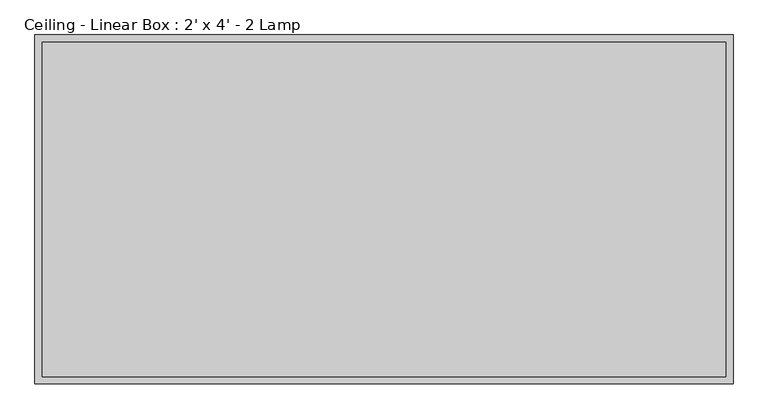
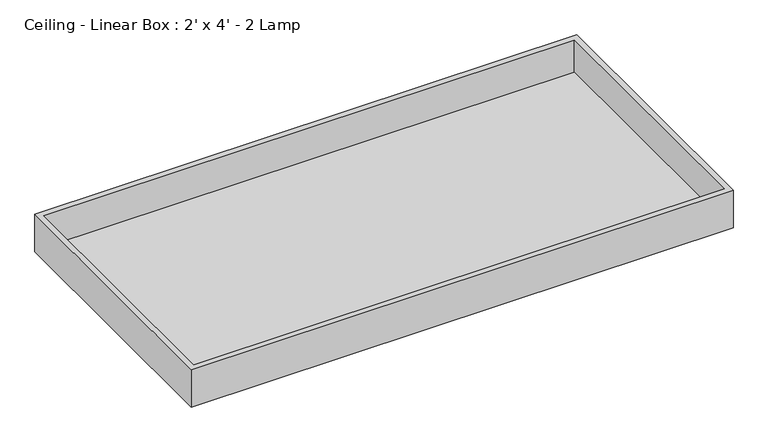
"""IFC4 building model written with IfcOpenShell, lengths in millimetres: light fixture geometry, Ceiling - Linear Box : 2' x 4' - 2 Lamp."""

import ifcopenshell
import ifcopenshell.guid

model = None  # the IFC model being written
_history = None  # IfcOwnerHistory: only IFC2X3 demands one
_inside = {}  # id of a spatial element -> (the spatial element, [elements in it])
_under = {}  # id of a project, library or spatial element -> (it, [spatial elements below it])
_declared = {}  # id of a project -> (the project, [libraries it declares])
_typed = {}  # id of a type object -> (the type object, [elements of that type])
_made_of = {}  # id of a material, layer set ... -> (it, [elements and type objects made of it])


def new_model(schema):
    """Start an empty IFC model of exactly this schema.

    Asked for "IFC4X3", IfcOpenShell would pick the latest addendum, in which some entities
    have other attributes; the version numbers below select the first issue.
    IFC2X3 requires an IfcOwnerHistory on every rooted entity: one is made here for all.
    """
    global model, _history
    if schema == "IFC4X3":
        model = ifcopenshell.file(schema_version=(4, 3, 0, 0))
    else:
        model = ifcopenshell.file(schema=schema)
    _inside.clear()
    _under.clear()
    _declared.clear()
    _typed.clear()
    _made_of.clear()
    _history = None
    if model.schema == "IFC2X3":
        org = make("IfcOrganization", Name="unknown")
        user = make(
            "IfcPersonAndOrganization",
            ThePerson=make("IfcPerson", FamilyName="unknown"),
            TheOrganization=org,
        )
        app = make(
            "IfcApplication",
            ApplicationDeveloper=org,
            Version="unknown",
            ApplicationFullName="unknown",
            ApplicationIdentifier="unknown",
        )
        _history = make(
            "IfcOwnerHistory",
            OwningUser=user,
            OwningApplication=app,
            ChangeAction="ADDED",
            CreationDate=0,
        )
    return model


def make(cls, **values):
    """One entity of the class cls with the attributes given. An attribute that is None is left unset."""
    return model.create_entity(
        cls, **{name: value for name, value in values.items() if value is not None}
    )


def rooted(cls, **values):
    """An entity with a GlobalId (a new one), such as an element, a storey or a relation."""
    return make(cls, GlobalId=ifcopenshell.guid.new(), OwnerHistory=_history, **values)


def si_unit(unit_type, name, prefix=None):
    """IfcSIUnit, for example si_unit("LENGTHUNIT", "METRE", prefix="MILLI")."""
    return make("IfcSIUnit", UnitType=unit_type, Prefix=prefix, Name=name)


def assignment(units):
    """IfcUnitAssignment: the units of a project."""
    return None if units is None else make("IfcUnitAssignment", Units=units)


def point(xyz):
    """IfcCartesianPoint."""
    return None if xyz is None else make("IfcCartesianPoint", Coordinates=xyz)


def direction(xyz):
    """IfcDirection."""
    return None if xyz is None else make("IfcDirection", DirectionRatios=xyz)


def frame(location, z_axis=None, x_axis=None):
    """IfcAxis2Placement3D, a coordinate frame: its origin and axes. An axis left out is left unset."""
    return make(
        "IfcAxis2Placement3D",
        Location=point(location),
        Axis=direction(z_axis),
        RefDirection=direction(x_axis),
    )


def origin():
    """The frame at (0, 0, 0) with its axes left unset."""
    return frame((0.0, 0.0, 0.0))


def place(relative_to, where):
    """IfcLocalPlacement: puts the frame where relative to a parent placement (None: the world)."""
    return make(
        "IfcLocalPlacement", PlacementRelTo=relative_to, RelativePlacement=where
    )


def context(
    kind, dimensions, precision=None, world=None, true_north=None, identifier=None
):
    """IfcGeometricRepresentationContext, for example the 3D "Model" context."""
    return make(
        "IfcGeometricRepresentationContext",
        ContextIdentifier=identifier,
        ContextType=kind,
        CoordinateSpaceDimension=dimensions,
        Precision=precision,
        WorldCoordinateSystem=world,
        TrueNorth=true_north,
    )


def project(units=None, contexts=None):
    """IfcProject with its units and contexts."""
    return rooted(
        "IfcProject",
        Name="project",
        RepresentationContexts=contexts,
        UnitsInContext=assignment(units),
    )


def spatial(cls, under=None, at=None, **own):
    """A site, building, storey or space (cls), placed at a placement, below another one or the project."""
    s = rooted(cls, ObjectPlacement=at, **own)
    if under is not None:
        _under.setdefault(under.id(), (under, []))[1].append(s)
    return s


def polyline(points):
    """IfcPolyline through the points."""
    return make("IfcPolyline", Points=[point(p) for p in points])


def outline(outer, holes=None, kind="AREA"):
    """IfcArbitraryClosedProfileDef: a profile drawn as a closed curve; with holes, ...WithVoids."""
    if holes is None:
        return make("IfcArbitraryClosedProfileDef", ProfileType=kind, OuterCurve=outer)
    return make(
        "IfcArbitraryProfileDefWithVoids",
        ProfileType=kind,
        OuterCurve=outer,
        InnerCurves=holes,
    )


def extrude(swept, where, along, depth):
    """IfcExtrudedAreaSolid: the profile swept, set in the frame where, extruded along a direction by depth."""
    return make(
        "IfcExtrudedAreaSolid",
        SweptArea=swept,
        Position=where,
        ExtrudedDirection=direction(along),
        Depth=depth,
    )


def shape(context_of_items, identifier, shape_type, items):
    """IfcShapeRepresentation: the items that make up one representation, for example the "Body"."""
    return make(
        "IfcShapeRepresentation",
        ContextOfItems=context_of_items,
        RepresentationIdentifier=identifier,
        RepresentationType=shape_type,
        Items=items,
    )


def source(mapping_origin, context_of_items, identifier, shape_type, items):
    """IfcRepresentationMap: a shape defined once, which mapped items show again and again."""
    return make(
        "IfcRepresentationMap",
        MappingOrigin=mapping_origin,
        MappedRepresentation=shape(context_of_items, identifier, shape_type, items),
    )


def transform(
    local_origin,
    x_axis=None,
    y_axis=None,
    z_axis=None,
    scale=None,
    scale2=None,
    scale3=None,
    uniform=True,
):
    """IfcCartesianTransformationOperator3D, or its non-uniform kind. x_axis, y_axis, z_axis: its Axis1, 2, 3."""
    if uniform:
        return make(
            "IfcCartesianTransformationOperator3D",
            Axis1=direction(x_axis),
            Axis2=direction(y_axis),
            LocalOrigin=point(local_origin),
            Scale=scale,
            Axis3=direction(z_axis),
        )
    return make(
        "IfcCartesianTransformationOperator3DnonUniform",
        Axis1=direction(x_axis),
        Axis2=direction(y_axis),
        LocalOrigin=point(local_origin),
        Scale=scale,
        Axis3=direction(z_axis),
        Scale2=scale2,
        Scale3=scale3,
    )


def mapped(mapping_source, mapping_target):
    """IfcMappedItem: shows the shape of a source again, moved by a transform."""
    return make(
        "IfcMappedItem", MappingSource=mapping_source, MappingTarget=mapping_target
    )


def made_of(thing, what):
    """Note that an element or type object is made of a material, layer set ...; save() writes the relation."""
    if what is not None:
        _made_of.setdefault(what.id(), (what, []))[1].append(thing)
    return thing


def element(
    cls,
    number,
    at=None,
    inside=None,
    cuts=None,
    type_object=None,
    material=None,
    context=None,
    identifier="Body",
    shape_type=None,
    held_by="IfcProductDefinitionShape",
    body=None,
    shapes=None,
    **own,
):
    """One element of the class cls, such as IfcWall. Its Tag is "e" and its number.

    at: its placement. inside: the storey or other place that contains it. cuts: it is an
    opening in that element (IfcRelVoidsElement). A single representation is given by context,
    identifier, shape_type and body (its items); several are given by shapes. held_by: the class
    of the entity that holds the representations. save() writes the other relations.
    """
    e = rooted(cls, Tag="e%d" % number, ObjectPlacement=at, **own)
    if body is not None:
        shapes = [shape(context, identifier, shape_type, body)]
    if shapes is not None:
        e.Representation = make(held_by, Representations=shapes)
    if inside is not None:
        _inside.setdefault(inside.id(), (inside, []))[1].append(e)
    if cuts is not None:
        rooted(
            "IfcRelVoidsElement", RelatingBuildingElement=cuts, RelatedOpeningElement=e
        )
    if type_object is not None:
        _typed.setdefault(type_object.id(), (type_object, []))[1].append(e)
    return made_of(e, material)


def aggregate(whole, parts):
    """IfcRelAggregates: a whole, such as a stair, and the parts it consists of."""
    return rooted("IfcRelAggregates", RelatingObject=whole, RelatedObjects=parts)


def save(model, path):
    """Write the relations noted so far, then the file.

    IfcRelAggregates (storeys below a building ...), IfcRelContainedInSpatialStructure (elements
    in a storey), IfcRelDefinesByType, IfcRelAssociatesMaterial and IfcRelDeclares: one each for
    every whole, place, type object, material and project.
    """
    for whole, parts in _under.values():
        aggregate(whole, parts)
    for where, things in _inside.values():
        rooted(
            "IfcRelContainedInSpatialStructure",
            RelatedElements=things,
            RelatingStructure=where,
        )
    for kind, things in _typed.values():
        rooted("IfcRelDefinesByType", RelatedObjects=things, RelatingType=kind)
    for what, things in _made_of.values():
        rooted("IfcRelAssociatesMaterial", RelatedObjects=things, RelatingMaterial=what)
    for by, libraries in _declared.values():
        rooted("IfcRelDeclares", RelatingContext=by, RelatedDefinitions=libraries)
    model.write(path)


def ceiling_linear_box_2_x_4_2_lamp_6471e3e8(model_context):
    return source(origin(), model_context, "Body", "SweptSolid", [
        extrude(outline(polyline([(596.9, 292.1), (596.9, -292.1), (-596.9, -292.1), (-596.9, 292.1), (596.9, 292.1)])), frame((0.0, 0.0, 2355.85), z_axis=(0.0, 0.0, 1.0), x_axis=(1.0, 0.0, 0.0)), (0.0, 0.0, 1.0), 6.35),
        extrude(outline(polyline([(609.6, 304.8), (609.6, -304.8), (-609.6, -304.8), (-609.6, 304.8), (609.6, 304.8)]), holes=[polyline([(596.9, 292.1), (-596.9, 292.1), (-596.9, -292.1), (596.9, -292.1), (596.9, 292.1)])]), frame((0.0, 0.0, 2349.5), z_axis=(0.0, 0.0, 1.0), x_axis=(1.0, 0.0, 0.0)), (0.0, 0.0, 1.0), 88.9),
    ])


if __name__ == "__main__":
    model = new_model("IFC4")
    model_context = context("Model", 3, world=origin())
    ifc_project = project(units=[si_unit("LENGTHUNIT", "METRE", prefix="MILLI")], contexts=[model_context])
    site = spatial("IfcSite", under=ifc_project)
    building = spatial("IfcBuilding", under=site)
    placement = place(None, origin())
    ceiling_linear_box_2_x_4_2_lamp_shape = ceiling_linear_box_2_x_4_2_lamp_6471e3e8(model_context)
    element("IfcLightFixture", 1, ObjectType="Ceiling - Linear Box : 2' x 4' - 2 Lamp", at=placement, inside=building, context=model_context, shape_type="MappedRepresentation", body=[
        mapped(ceiling_linear_box_2_x_4_2_lamp_shape, transform((0.0, 0.0, 0.0), x_axis=(1.0, 0.0, 0.0), y_axis=(0.0, 1.0, 0.0), z_axis=(0.0, 0.0, 1.0))),
    ])
    save(model, "model.ifc")

# Revit data of these elements
# Type "Ceiling - Linear Box : 2' x 4' - 2 Lamp"
#   Assembly Code = "D5020210"
#   Lamp = "T-12"
#   Wattage = 32.3141 W
#   built-in parameter 1150110 = 1 (stored number, unit not read)
#   built-in parameter 1114217 = 1 (stored number, unit not read)
#   built-in parameter 1150109 = 1 (stored number, unit not read)
#   built-in parameter 1150113 = 1 (stored number, unit not read)
#   built-in parameter 1150105 = 381.972 (stored number, unit not read)
#   built-in parameter 1150115 = 1 (stored number, unit not read)
#   Light Source Symbol Size = 2' - 0"
#   built-in parameter 1150112 = 1 (stored number, unit not read)
#   built-in parameter 1150114 = 1 (stored number, unit not read)
#   built-in parameter 1150107 = 3200 (stored number, unit not read)
#   built-in parameter 1150106 = 3.81972 (stored number, unit not read)
#   Emit from Line Length = 2' - 0"
#   built-in parameter 1150104 = 13.8 (stored number, unit not read)
#   built-in parameter 1114218 = 1 (stored number, unit not read)
#   built-in parameter 1150133 = 10 (stored number, unit not read)
#   Length = 4' - 0"
#   Lumens = 4800 lm
#   Width = 2' - 0"
#   built-in parameter 1150134 = 3
#   built-in parameter 1150132 = 2
#   Color Filter = 16777215
#   Diffuser = none
#   Light Box = none
#   Dimming Lamp Color Temperature Shift = (empty or 0)
